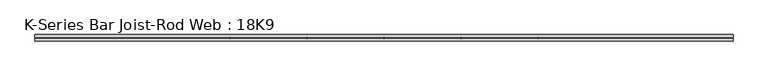
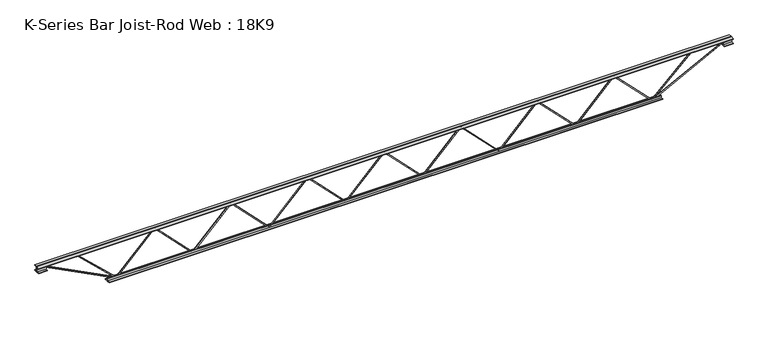
"""IFC4 building model written with IfcOpenShell, lengths in millimetres: beam geometry, K-Series Bar Joist-Rod Web : 18K9."""

from ifc_helpers import new_model, si_unit, frame, origin, place, context, project, spatial, polyline, outline, extrude, source, transform, mapped, element, save


def k_series_bar_joist_rod_web_18k9_87758491(model_context):
    return source(origin(), model_context, "Body", "SweptSolid", [
        extrude(outline(polyline([(-217.4875, 1323.6348214), (-227.0125, 1323.6348214), (-227.0125, 1328.8131603), (217.4875, 1763.6747675), (217.4875, 1766.0180897), (-227.0125, 2200.8796968), (-227.0125, 2206.0580357), (-217.4875, 2206.0580357), (-217.4875, 2204.8863746), (227.0125, 1770.0247675), (227.0125, 1759.6680897), (-217.4875, 1324.8064825), (-217.4875, 1323.6348214)])), frame((0.0, -4.7625, 0.0), z_axis=(0.0, 1.0, 0.0), x_axis=(0.0, 0.0, 1.0)), (0.0, 0.0, 1.0), 9.525),
        extrude(outline(polyline([(-217.4875, 441.2116071), (-227.0125, 441.2116071), (-227.0125, 446.389946), (217.4875, 881.2515532), (217.4875, 883.5948754), (-227.0125, 1318.4564825), (-227.0125, 1323.6348214), (-217.4875, 1323.6348214), (-217.4875, 1322.4631603), (227.0125, 887.6015532), (227.0125, 877.2448754), (-217.4875, 442.3832682), (-217.4875, 441.2116071)])), frame((0.0, -4.7625, 0.0), z_axis=(0.0, 1.0, 0.0), x_axis=(0.0, 0.0, 1.0)), (0.0, 0.0, 1.0), 9.525),
        extrude(outline(polyline([(-217.4875, -441.2116071), (-227.0125, -441.2116071), (-227.0125, -436.0332682), (217.4875, -1.1716611), (217.4875, 1.1716611), (-227.0125, 436.0332682), (-227.0125, 441.2116071), (-217.4875, 441.2116071), (-217.4875, 440.039946), (227.0125, 5.1783389), (227.0125, -5.1783389), (-217.4875, -440.039946), (-217.4875, -441.2116071)])), frame((0.0, -4.7625, 0.0), z_axis=(0.0, 1.0, 0.0), x_axis=(0.0, 0.0, 1.0)), (0.0, 0.0, 1.0), 9.525),
        extrude(outline(polyline([(-217.4875, -1323.6348214), (-227.0125, -1323.6348214), (-227.0125, -1318.4564825), (217.4875, -883.5948754), (217.4875, -881.2515532), (-227.0125, -446.389946), (-227.0125, -441.2116071), (-217.4875, -441.2116071), (-217.4875, -442.3832682), (227.0125, -877.2448754), (227.0125, -887.6015532), (-217.4875, -1322.4631603), (-217.4875, -1323.6348214)])), frame((0.0, -4.7625, 0.0), z_axis=(0.0, 1.0, 0.0), x_axis=(0.0, 0.0, 1.0)), (0.0, 0.0, 1.0), 9.525),
        extrude(outline(polyline([(-217.4875, -2206.0580357), (-227.0125, -2206.0580357), (-227.0125, -2200.8796968), (217.4875, -1766.0180897), (217.4875, -1763.6747675), (-227.0125, -1328.8131603), (-227.0125, -1323.6348214), (-217.4875, -1323.6348214), (-217.4875, -1324.8064825), (227.0125, -1759.6680897), (227.0125, -1770.0247675), (-217.4875, -2204.8863746), (-217.4875, -2206.0580357)])), frame((0.0, -4.7625, 0.0), z_axis=(0.0, 1.0, 0.0), x_axis=(0.0, 0.0, 1.0)), (0.0, 0.0, 1.0), 9.525),
        extrude(outline(polyline([(-217.4875, 2206.0580357), (-227.0125, 2206.0580357), (-227.0125, 2211.2363746), (217.4875, 2646.0979818), (217.4875, 2648.441304), (-227.0125, 3083.3029111), (-227.0125, 3088.48125), (-217.4875, 3088.48125), (-217.4875, 3087.3095889), (227.0125, 2652.4479818), (227.0125, 2642.091304), (-217.4875, 2207.2296968), (-217.4875, 2206.0580357)])), frame((0.0, -4.7625, 0.0), z_axis=(0.0, 1.0, 0.0), x_axis=(0.0, 0.0, 1.0)), (0.0, 0.0, 1.0), 9.525),
        extrude(outline(polyline([(-217.4875, -3088.48125), (-227.0125, -3088.48125), (-227.0125, -3083.3029111), (217.4875, -2648.441304), (217.4875, -2646.0979818), (-227.0125, -2211.2363746), (-227.0125, -2206.0580357), (-217.4875, -2206.0580357), (-217.4875, -2207.2296968), (227.0125, -2642.091304), (227.0125, -2652.4479818), (-217.4875, -3087.3095889), (-217.4875, -3088.48125)])), frame((0.0, -4.7625, 0.0), z_axis=(0.0, 1.0, 0.0), x_axis=(0.0, 0.0, 1.0)), (0.0, 0.0, 1.0), 9.525),
        extrude(outline(polyline([(4.7625, 228.6), (36.5125, 228.6), (36.5125, 222.25), (11.1125, 222.25), (11.1125, 196.85), (4.7625, 196.85), (4.7625, 228.6)])), frame((-4002.88125, 0.0, 0.0), z_axis=(1.0, 0.0, 0.0), x_axis=(0.0, 1.0, 0.0)), (0.0, 0.0, 1.0), 8005.7625),
        extrude(outline(polyline([(-4.7625, 228.6), (-4.7625, 196.85), (-11.1125, 196.85), (-11.1125, 222.25), (-36.5125, 222.25), (-36.5125, 228.6), (-4.7625, 228.6)])), frame((-4002.88125, 0.0, 0.0), z_axis=(1.0, 0.0, 0.0), x_axis=(0.0, 1.0, 0.0)), (0.0, 0.0, 1.0), 8005.7625),
        extrude(outline(polyline([(-4.7625, 165.1), (-36.5125, 165.1), (-36.5125, 171.45), (-11.1125, 171.45), (-11.1125, 196.85), (-4.7625, 196.85), (-4.7625, 165.1)])), frame((-4002.88125, 0.0, 0.0), z_axis=(1.0, 0.0, 0.0), x_axis=(0.0, 1.0, 0.0)), (0.0, 0.0, 1.0), 101.6),
        extrude(outline(polyline([(36.5125, 165.1), (4.7625, 165.1), (4.7625, 196.85), (11.1125, 196.85), (11.1125, 171.45), (36.5125, 171.45), (36.5125, 165.1)])), frame((-4002.88125, 0.0, 0.0), z_axis=(1.0, 0.0, 0.0), x_axis=(0.0, 1.0, 0.0)), (0.0, 0.0, 1.0), 101.6),
        extrude(outline(polyline([(4.7625, 165.1), (4.7625, 196.85), (11.1125, 196.85), (11.1125, 171.45), (36.5125, 171.45), (36.5125, 165.1), (4.7625, 165.1)])), frame((3901.28125, 0.0, 0.0), z_axis=(1.0, 0.0, 0.0), x_axis=(0.0, 1.0, 0.0)), (0.0, 0.0, 1.0), 101.6),
        extrude(outline(polyline([(-4.7625, 165.1), (-36.5125, 165.1), (-36.5125, 171.45), (-11.1125, 171.45), (-11.1125, 196.85), (-4.7625, 196.85), (-4.7625, 165.1)])), frame((3901.28125, 0.0, 0.0), z_axis=(1.0, 0.0, 0.0), x_axis=(0.0, 1.0, 0.0)), (0.0, 0.0, 1.0), 101.6),
        extrude(outline(polyline([(4.7625, -228.6), (4.7625, -196.85), (11.1125, -196.85), (11.1125, -222.25), (36.5125, -222.25), (36.5125, -228.6), (4.7625, -228.6)])), frame((-3190.08125, 0.0, 0.0), z_axis=(1.0, 0.0, 0.0), x_axis=(0.0, 1.0, 0.0)), (0.0, 0.0, 1.0), 6380.1625),
        extrude(outline(polyline([(-4.7625, -228.6), (-36.5125, -228.6), (-36.5125, -222.25), (-11.1125, -222.25), (-11.1125, -196.85), (-4.7625, -196.85), (-4.7625, -228.6)])), frame((-3190.08125, 0.0, 0.0), z_axis=(1.0, 0.0, 0.0), x_axis=(0.0, 1.0, 0.0)), (0.0, 0.0, 1.0), 6380.1625),
        extrude(outline(polyline([(0.0, -9.525), (0.0, 0.0), (914.4881902, 0.0), (914.4881902, -9.525), (0.0, -9.525)])), frame((-3903.463852, 4.7625, 192.6170749), z_axis=(0.45828913319472675, 0.0, 0.8888031674086373), x_axis=(0.8888031674086373, 0.0, -0.45828913319472675)), (0.0, 0.0, 1.0), 9.525),
        extrude(outline(polyline([(0.0, -9.525), (0.0, 0.0), (608.5330659, 0.0), (608.5330659, -9.525), (0.0, -9.525)])), frame((-3532.9728165, 4.7625, 193.3969908), z_axis=(0.6887053859416878, 0.0, 0.725041303219969), x_axis=(0.725041303219969, 0.0, -0.6887053859416878)), (0.0, 0.0, 1.0), 9.525),
        extrude(outline(polyline([(0.0, -9.525), (0.0, 0.0), (914.4881902, 0.0), (914.4881902, -9.525), (0.0, -9.525)])), frame((3903.463852, -4.7625, 192.6170749), z_axis=(-0.4582891331947156, 0.0, 0.8888031674086431), x_axis=(-0.8888031674086431, 0.0, -0.4582891331947156)), (0.0, 0.0, 1.0), 9.525),
        extrude(outline(polyline([(0.0, -9.525), (0.0, 0.0), (608.5330659, 0.0), (608.5330659, -9.525), (0.0, -9.525)])), frame((3532.9728165, -4.7625, 193.3969908), z_axis=(-0.6887053859416835, 0.0, 0.725041303219973), x_axis=(-0.725041303219973, 0.0, -0.6887053859416835)), (0.0, 0.0, 1.0), 9.525),
    ])


if __name__ == "__main__":
    model = new_model("IFC4")
    model_context = context("Model", 3, world=origin())
    ifc_project = project(units=[si_unit("LENGTHUNIT", "METRE", prefix="MILLI")], contexts=[model_context])
    site = spatial("IfcSite", under=ifc_project)
    building = spatial("IfcBuilding", under=site)
    placement = place(None, origin())
    k_series_bar_joist_rod_web_18k9_shape = k_series_bar_joist_rod_web_18k9_87758491(model_context)
    element("IfcBeam", 1, ObjectType="K-Series Bar Joist-Rod Web : 18K9", at=placement, inside=building, context=model_context, shape_type="MappedRepresentation", body=[
        mapped(k_series_bar_joist_rod_web_18k9_shape, transform((0.0, 0.0, 0.0), x_axis=(1.0, 0.0, 0.0), y_axis=(0.0, 1.0, 0.0), z_axis=(0.0, 0.0, 1.0))),
    ])
    save(model, "model.ifc")

# Revit data of these elements
# Type "K-Series Bar Joist-Rod Web : 18K9"
#   Assembly Code = "B1010350"
#   Wt = 10.2
#   Web Thickness = 0' - 0 3/8"
#   Start Offset [instance default] = 0' - 0"
#   Start Extension [instance default] = 0' - 0"
#   Seat Length = 0' - 4"
#   Seat Depth = 0' - 2 1/2"
#   PanelArrayLength [instance default] = 18' - 0"
#   Panel [instance default] = 3' - 0"
#   End Offset [instance default] = 0' - 0"
#   End Extension [instance default] = 0' - 0"
#   End Panel = 3' - 0"
#   Cord Leg = 0' - 1 1/4"
#   Chord Thickness = 0' - 0 1/4"
#   Length [instance default] = 24' - 0"
#   Depth = 1' - 6"
#   PanelArrayNum [instance default] = 6
#   Structural Material = none
# Element 1 (IfcBeam, "K-Series Bar Joist-Rod Web : 18K9")
#   PanelArrayLength = 20' - 3 3/16"
#   Panel = 2' - 10.74107"
#   PanelArrayNum = 7
